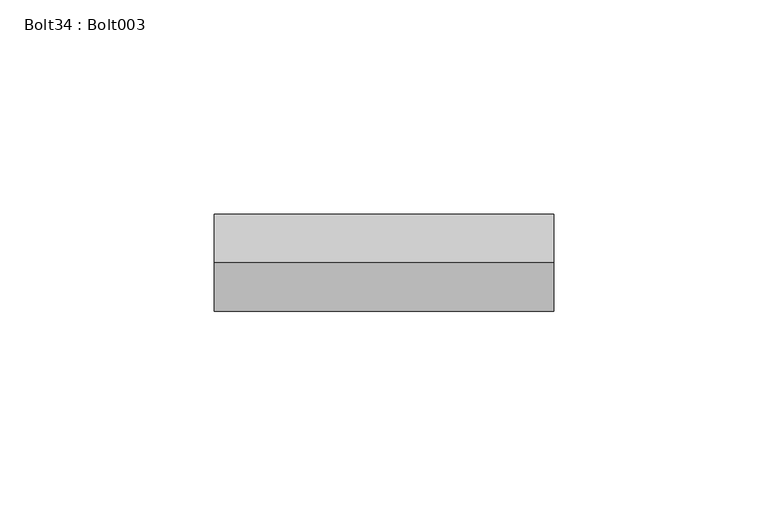
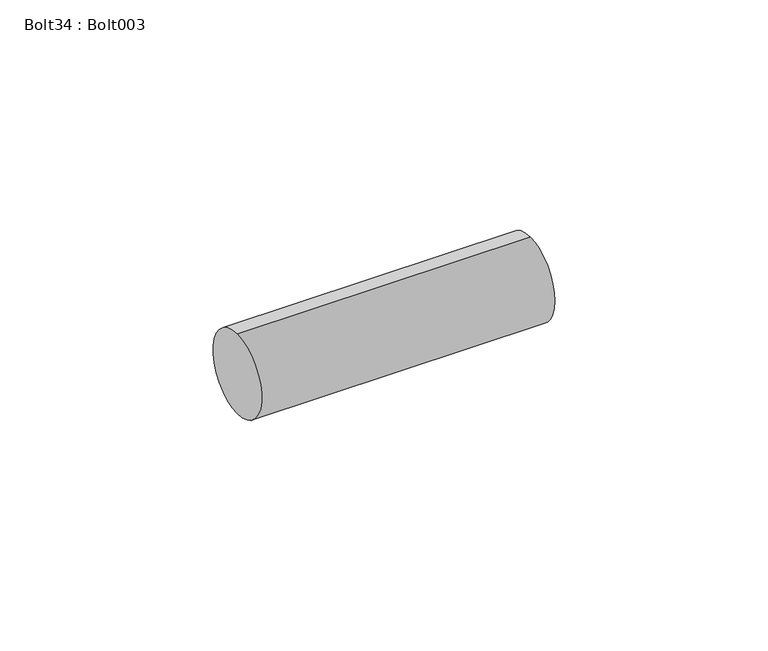
"""IFC4 building model written with IfcOpenShell, lengths in millimetres: proxy geometry, Bolt34 : Bolt003."""

import ifcopenshell
import ifcopenshell.guid

model = None  # the IFC model being written
_history = None  # IfcOwnerHistory: only IFC2X3 demands one
_inside = {}  # id of a spatial element -> (the spatial element, [elements in it])
_under = {}  # id of a project, library or spatial element -> (it, [spatial elements below it])
_declared = {}  # id of a project -> (the project, [libraries it declares])
_typed = {}  # id of a type object -> (the type object, [elements of that type])
_made_of = {}  # id of a material, layer set ... -> (it, [elements and type objects made of it])


def new_model(schema):
    """Start an empty IFC model of exactly this schema.

    Asked for "IFC4X3", IfcOpenShell would pick the latest addendum, in which some entities
    have other attributes; the version numbers below select the first issue.
    IFC2X3 requires an IfcOwnerHistory on every rooted entity: one is made here for all.
    """
    global model, _history
    if schema == "IFC4X3":
        model = ifcopenshell.file(schema_version=(4, 3, 0, 0))
    else:
        model = ifcopenshell.file(schema=schema)
    _inside.clear()
    _under.clear()
    _declared.clear()
    _typed.clear()
    _made_of.clear()
    _history = None
    if model.schema == "IFC2X3":
        org = make("IfcOrganization", Name="unknown")
        user = make(
            "IfcPersonAndOrganization",
            ThePerson=make("IfcPerson", FamilyName="unknown"),
            TheOrganization=org,
        )
        app = make(
            "IfcApplication",
            ApplicationDeveloper=org,
            Version="unknown",
            ApplicationFullName="unknown",
            ApplicationIdentifier="unknown",
        )
        _history = make(
            "IfcOwnerHistory",
            OwningUser=user,
            OwningApplication=app,
            ChangeAction="ADDED",
            CreationDate=0,
        )
    return model


def make(cls, **values):
    """One entity of the class cls with the attributes given. An attribute that is None is left unset."""
    return model.create_entity(
        cls, **{name: value for name, value in values.items() if value is not None}
    )


def rooted(cls, **values):
    """An entity with a GlobalId (a new one), such as an element, a storey or a relation."""
    return make(cls, GlobalId=ifcopenshell.guid.new(), OwnerHistory=_history, **values)


def si_unit(unit_type, name, prefix=None):
    """IfcSIUnit, for example si_unit("LENGTHUNIT", "METRE", prefix="MILLI")."""
    return make("IfcSIUnit", UnitType=unit_type, Prefix=prefix, Name=name)


def assignment(units):
    """IfcUnitAssignment: the units of a project."""
    return None if units is None else make("IfcUnitAssignment", Units=units)


def point(xyz):
    """IfcCartesianPoint."""
    return None if xyz is None else make("IfcCartesianPoint", Coordinates=xyz)


def direction(xyz):
    """IfcDirection."""
    return None if xyz is None else make("IfcDirection", DirectionRatios=xyz)


def frame(location, z_axis=None, x_axis=None):
    """IfcAxis2Placement3D, a coordinate frame: its origin and axes. An axis left out is left unset."""
    return make(
        "IfcAxis2Placement3D",
        Location=point(location),
        Axis=direction(z_axis),
        RefDirection=direction(x_axis),
    )


def frame_2d(location, x_axis=None):
    """IfcAxis2Placement2D, a coordinate frame in the plane: its origin and x axis."""
    return make(
        "IfcAxis2Placement2D", Location=point(location), RefDirection=direction(x_axis)
    )


def origin():
    """The frame at (0, 0, 0) with its axes left unset."""
    return frame((0.0, 0.0, 0.0))


def place(relative_to, where):
    """IfcLocalPlacement: puts the frame where relative to a parent placement (None: the world)."""
    return make(
        "IfcLocalPlacement", PlacementRelTo=relative_to, RelativePlacement=where
    )


def context(
    kind, dimensions, precision=None, world=None, true_north=None, identifier=None
):
    """IfcGeometricRepresentationContext, for example the 3D "Model" context."""
    return make(
        "IfcGeometricRepresentationContext",
        ContextIdentifier=identifier,
        ContextType=kind,
        CoordinateSpaceDimension=dimensions,
        Precision=precision,
        WorldCoordinateSystem=world,
        TrueNorth=true_north,
    )


def project(units=None, contexts=None):
    """IfcProject with its units and contexts."""
    return rooted(
        "IfcProject",
        Name="project",
        RepresentationContexts=contexts,
        UnitsInContext=assignment(units),
    )


def spatial(cls, under=None, at=None, **own):
    """A site, building, storey or space (cls), placed at a placement, below another one or the project."""
    s = rooted(cls, ObjectPlacement=at, **own)
    if under is not None:
        _under.setdefault(under.id(), (under, []))[1].append(s)
    return s


def circle_curve(where, radius):
    """IfcCircle in the frame where."""
    return make("IfcCircle", Position=where, Radius=radius)


def trimmed(basis, trim1, trim2, sense, master):
    """IfcTrimmedCurve: the piece of a basis curve between two trims."""
    return make(
        "IfcTrimmedCurve",
        BasisCurve=basis,
        Trim1=trim1,
        Trim2=trim2,
        SenseAgreement=sense,
        MasterRepresentation=master,
    )


def segment(curve, same_sense, transition):
    """IfcCompositeCurveSegment."""
    return make(
        "IfcCompositeCurveSegment",
        Transition=transition,
        SameSense=same_sense,
        ParentCurve=curve,
    )


def composite_curve(segments, self_intersect=None):
    """IfcCompositeCurve: segments joined end to end."""
    return make("IfcCompositeCurve", Segments=segments, SelfIntersect=self_intersect)


def outline(outer, holes=None, kind="AREA"):
    """IfcArbitraryClosedProfileDef: a profile drawn as a closed curve; with holes, ...WithVoids."""
    if holes is None:
        return make("IfcArbitraryClosedProfileDef", ProfileType=kind, OuterCurve=outer)
    return make(
        "IfcArbitraryProfileDefWithVoids",
        ProfileType=kind,
        OuterCurve=outer,
        InnerCurves=holes,
    )


def extrude(swept, where, along, depth):
    """IfcExtrudedAreaSolid: the profile swept, set in the frame where, extruded along a direction by depth."""
    return make(
        "IfcExtrudedAreaSolid",
        SweptArea=swept,
        Position=where,
        ExtrudedDirection=direction(along),
        Depth=depth,
    )


def shape(context_of_items, identifier, shape_type, items):
    """IfcShapeRepresentation: the items that make up one representation, for example the "Body"."""
    return make(
        "IfcShapeRepresentation",
        ContextOfItems=context_of_items,
        RepresentationIdentifier=identifier,
        RepresentationType=shape_type,
        Items=items,
    )


def source(mapping_origin, context_of_items, identifier, shape_type, items):
    """IfcRepresentationMap: a shape defined once, which mapped items show again and again."""
    return make(
        "IfcRepresentationMap",
        MappingOrigin=mapping_origin,
        MappedRepresentation=shape(context_of_items, identifier, shape_type, items),
    )


def transform(
    local_origin,
    x_axis=None,
    y_axis=None,
    z_axis=None,
    scale=None,
    scale2=None,
    scale3=None,
    uniform=True,
):
    """IfcCartesianTransformationOperator3D, or its non-uniform kind. x_axis, y_axis, z_axis: its Axis1, 2, 3."""
    if uniform:
        return make(
            "IfcCartesianTransformationOperator3D",
            Axis1=direction(x_axis),
            Axis2=direction(y_axis),
            LocalOrigin=point(local_origin),
            Scale=scale,
            Axis3=direction(z_axis),
        )
    return make(
        "IfcCartesianTransformationOperator3DnonUniform",
        Axis1=direction(x_axis),
        Axis2=direction(y_axis),
        LocalOrigin=point(local_origin),
        Scale=scale,
        Axis3=direction(z_axis),
        Scale2=scale2,
        Scale3=scale3,
    )


def mapped(mapping_source, mapping_target):
    """IfcMappedItem: shows the shape of a source again, moved by a transform."""
    return make(
        "IfcMappedItem", MappingSource=mapping_source, MappingTarget=mapping_target
    )


def made_of(thing, what):
    """Note that an element or type object is made of a material, layer set ...; save() writes the relation."""
    if what is not None:
        _made_of.setdefault(what.id(), (what, []))[1].append(thing)
    return thing


def element(
    cls,
    number,
    at=None,
    inside=None,
    cuts=None,
    type_object=None,
    material=None,
    context=None,
    identifier="Body",
    shape_type=None,
    held_by="IfcProductDefinitionShape",
    body=None,
    shapes=None,
    **own,
):
    """One element of the class cls, such as IfcWall. Its Tag is "e" and its number.

    at: its placement. inside: the storey or other place that contains it. cuts: it is an
    opening in that element (IfcRelVoidsElement). A single representation is given by context,
    identifier, shape_type and body (its items); several are given by shapes. held_by: the class
    of the entity that holds the representations. save() writes the other relations.
    """
    e = rooted(cls, Tag="e%d" % number, ObjectPlacement=at, **own)
    if body is not None:
        shapes = [shape(context, identifier, shape_type, body)]
    if shapes is not None:
        e.Representation = make(held_by, Representations=shapes)
    if inside is not None:
        _inside.setdefault(inside.id(), (inside, []))[1].append(e)
    if cuts is not None:
        rooted(
            "IfcRelVoidsElement", RelatingBuildingElement=cuts, RelatedOpeningElement=e
        )
    if type_object is not None:
        _typed.setdefault(type_object.id(), (type_object, []))[1].append(e)
    return made_of(e, material)


def aggregate(whole, parts):
    """IfcRelAggregates: a whole, such as a stair, and the parts it consists of."""
    return rooted("IfcRelAggregates", RelatingObject=whole, RelatedObjects=parts)


def save(model, path):
    """Write the relations noted so far, then the file.

    IfcRelAggregates (storeys below a building ...), IfcRelContainedInSpatialStructure (elements
    in a storey), IfcRelDefinesByType, IfcRelAssociatesMaterial and IfcRelDeclares: one each for
    every whole, place, type object, material and project.
    """
    for whole, parts in _under.values():
        aggregate(whole, parts)
    for where, things in _inside.values():
        rooted(
            "IfcRelContainedInSpatialStructure",
            RelatedElements=things,
            RelatingStructure=where,
        )
    for kind, things in _typed.values():
        rooted("IfcRelDefinesByType", RelatedObjects=things, RelatingType=kind)
    for what, things in _made_of.values():
        rooted("IfcRelAssociatesMaterial", RelatedObjects=things, RelatingMaterial=what)
    for by, libraries in _declared.values():
        rooted("IfcRelDeclares", RelatingContext=by, RelatedDefinitions=libraries)
    model.write(path)


def bolt34_bolt003_4129b6dc(model_context):
    return source(origin(), model_context, "Body", "SweptSolid", [
        extrude(outline(composite_curve([segment(trimmed(circle_curve(frame_2d((1896.5882072, 40070.0545241)), 11.4045168), [point((1896.5882072, 40058.6500073))], [point((1896.5882072, 40081.4590409))], False, "CARTESIAN"), True, "CONTINUOUS"), segment(trimmed(circle_curve(frame_2d((1896.5882072, 40070.0545241)), 11.4045168), [point((1896.5882072, 40081.4590409))], [point((1896.5882072, 40058.6500073))], False, "CARTESIAN"), True, "CONTINUOUS")], self_intersect=False)), frame((10265.0890809, 0.0, 0.0), z_axis=(1.0, 0.0, 0.0), x_axis=(0.0, 1.0, 0.0)), (0.0, 0.0, 1.0), 79.375),
    ])


if __name__ == "__main__":
    model = new_model("IFC4")
    model_context = context("Model", 3, world=origin())
    ifc_project = project(units=[si_unit("LENGTHUNIT", "METRE", prefix="MILLI")], contexts=[model_context])
    site = spatial("IfcSite", under=ifc_project)
    building = spatial("IfcBuilding", under=site)
    placement = place(None, origin())
    bolt34_bolt003_shape = bolt34_bolt003_4129b6dc(model_context)
    element("IfcBuildingElementProxy", 1, Name="Bolt34 : Bolt003", ObjectType="Bolt34 : Bolt003", at=placement, inside=building, context=model_context, shape_type="MappedRepresentation", body=[
        mapped(bolt34_bolt003_shape, transform((0.0, 0.0, 0.0), x_axis=(1.0, 0.0, 0.0), y_axis=(0.0, 1.0, 0.0), z_axis=(0.0, 0.0, 1.0))),
    ])
    save(model, "model.ifc")

# Revit data of these elements
# Type "Bolt34 : Bolt003"
#   NameOverride = "Bolt003"
# Element 1 (IfcBuildingElementProxy, "Bolt34 : Bolt003")
#   Materials on its faces: "STEEL ANGLE AND ANCHOR BOLT (SEE STRUCT. DWGS)"
# Materials
#   "STEEL ANGLE AND ANCHOR BOLT (SEE STRUCT. DWGS)": class "Unassigned", colour RGB 128 128 128, transparency 0, Cost = 0
